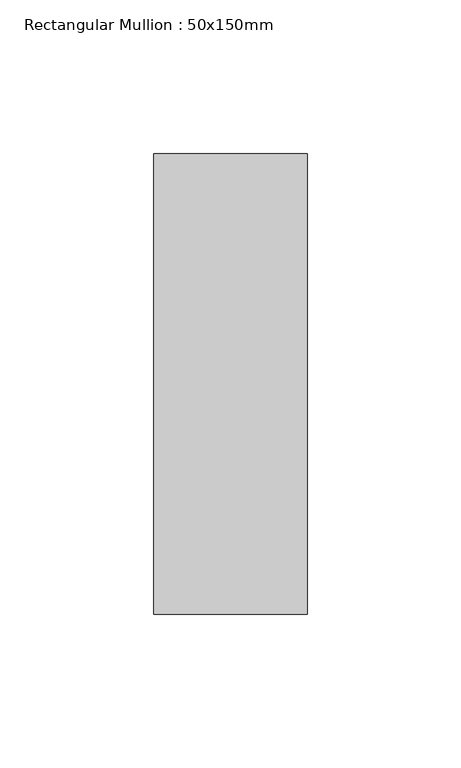
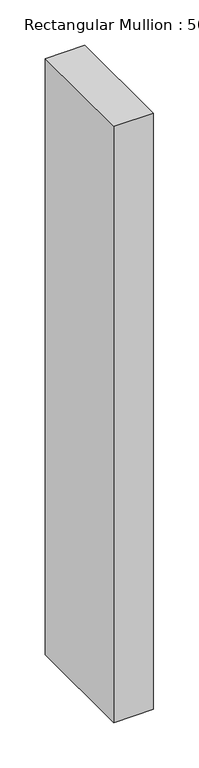
"""IFC4 building model written with IfcOpenShell, lengths in millimetres: member geometry, Rectangular Mullion : 50x150mm."""

from ifc_helpers import new_model, si_unit, frame, origin, place, context, project, spatial, polyline, outline, extrude, source, transform, mapped, element, save


def rectangular_mullion_50x150mm_6ffebc0f(model_context):
    return source(origin(), model_context, "Body", "SweptSolid", [
        extrude(outline(polyline([(0.0, 75.0), (0.0, -75.0), (-50.0, -75.0), (-50.0, 75.0), (0.0, 75.0)])), frame((0.0, 0.0, -800.0), z_axis=(0.0, 0.0, 1.0), x_axis=(1.0, 0.0, 0.0)), (0.0, 0.0, 1.0), 800.0),
    ])


if __name__ == "__main__":
    model = new_model("IFC4")
    model_context = context("Model", 3, world=origin())
    ifc_project = project(units=[si_unit("LENGTHUNIT", "METRE", prefix="MILLI")], contexts=[model_context])
    site = spatial("IfcSite", under=ifc_project)
    building = spatial("IfcBuilding", under=site)
    placement = place(None, origin())
    rectangular_mullion_50x150mm_shape = rectangular_mullion_50x150mm_6ffebc0f(model_context)
    element("IfcMember", 1, ObjectType="Rectangular Mullion : 50x150mm", at=placement, inside=building, context=model_context, shape_type="MappedRepresentation", body=[
        mapped(rectangular_mullion_50x150mm_shape, transform((0.0, 0.0, 0.0), x_axis=(1.0, 0.0, 0.0), y_axis=(0.0, 1.0, 0.0), z_axis=(0.0, 0.0, 1.0))),
    ])
    save(model, "model.ifc")

# Revit data of these elements
# Type "Rectangular Mullion : 50x150mm"
#   Keynote = "H11"
#   built-in parameter 1007304 = 0.492126 (stored number, unit not read)
#   built-in parameter 1007301 = 0.082021 (stored number, unit not read)
#   built-in parameter 1007300 = 0.082021 (stored number, unit not read)
# Element 1 (IfcMember, "Rectangular Mullion : 50x150mm")
#   Materials on its faces: "Aluminium"
# Materials
#   "Aluminium": class "Metal", colour RGB 247 247 247, transparency 0, Description = "Aluminium 6061", Cost = 0
